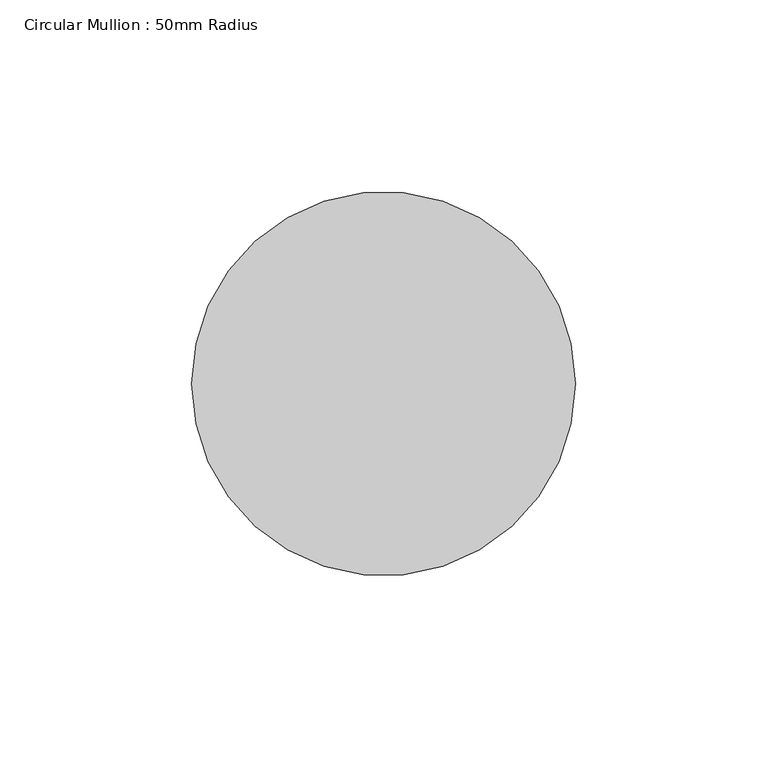
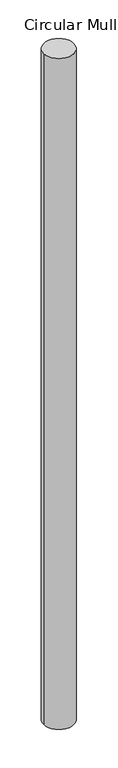
"""IFC4 building model written with IfcOpenShell, lengths in millimetres: member geometry, Circular Mullion : 50mm Radius."""

from ifc_helpers import new_model, si_unit, point, frame, frame_2d, origin, place, context, project, spatial, circle_curve, trimmed, segment, composite_curve, outline, extrude, source, transform, mapped, element, save


def circular_mullion_50mm_radius_a5e5482e(model_context):
    return source(origin(), model_context, "Body", "SweptSolid", [
        extrude(outline(composite_curve([segment(trimmed(circle_curve(frame_2d((-50.0, 0.0)), 50.0), [point((0.0, 0.0))], [point((-100.0, 0.0))], False, "CARTESIAN"), True, "CONTINUOUS"), segment(trimmed(circle_curve(frame_2d((-50.0, 0.0)), 50.0), [point((-100.0, 0.0))], [point((0.0, 0.0))], False, "CARTESIAN"), True, "CONTINUOUS")], self_intersect=False)), frame((0.0, 0.0, -2340.6926851), z_axis=(0.0, 0.0, 1.0), x_axis=(1.0, 0.0, 0.0)), (0.0, 0.0, 1.0), 2340.6926851),
    ])


if __name__ == "__main__":
    model = new_model("IFC4")
    model_context = context("Model", 3, world=origin())
    ifc_project = project(units=[si_unit("LENGTHUNIT", "METRE", prefix="MILLI")], contexts=[model_context])
    site = spatial("IfcSite", under=ifc_project)
    building = spatial("IfcBuilding", under=site)
    placement = place(None, origin())
    circular_mullion_50mm_radius_shape = circular_mullion_50mm_radius_a5e5482e(model_context)
    element("IfcMember", 1, ObjectType="Circular Mullion : 50mm Radius", at=placement, inside=building, context=model_context, shape_type="MappedRepresentation", body=[
        mapped(circular_mullion_50mm_radius_shape, transform((0.0, 0.0, 0.0), x_axis=(1.0, 0.0, 0.0), y_axis=(0.0, 1.0, 0.0), z_axis=(0.0, 0.0, 1.0))),
    ])
    save(model, "model.ifc")

# Revit data of these elements
# Type "Circular Mullion : 50mm Radius"
#   built-in parameter 1007350 = 0.164042 (stored number, unit not read)
# Element 1 (IfcMember, "Circular Mullion : 50mm Radius")
#   Materials on its faces: "Aluminium"
# Materials
#   "Aluminium": class "Metal", colour RGB 247 247 247, transparency 0, Description = "Aluminium 6061", Cost = 0
